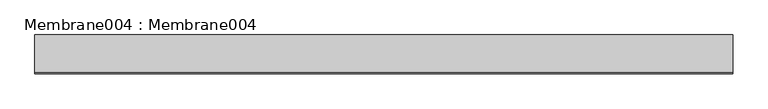
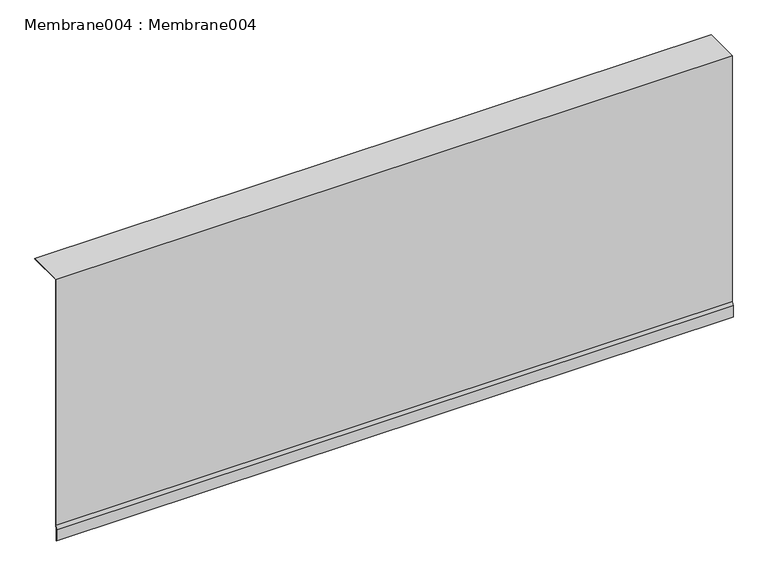
"""IFC4 building model written with IfcOpenShell, lengths in millimetres: proxy geometry, Membrane004 : Membrane004."""

from ifc_helpers import new_model, si_unit, frame, origin, place, context, project, spatial, polyline, outline, extrude, source, transform, mapped, element, save


def membrane004_membrane004_f78f7f05(model_context):
    return source(origin(), model_context, "Body", "SweptSolid", [
        extrude(outline(polyline([(-4304.4792138, 41057.992875), (-4304.4792138, 41056.992875), (-4410.2786824, 41056.992875), (-4410.2786824, 40289.0915624), (-4414.3643448, 40277.8662972), (-4414.3643448, 40242.9648437), (-4415.3643448, 40242.9648437), (-4415.3643448, 40278.0426242), (-4411.2786824, 40289.2678894), (-4411.2786824, 41057.992875), (-4304.4792138, 41057.992875)])), frame((12383.0178845, 0.0, 0.0), z_axis=(1.0, 0.0, 0.0), x_axis=(0.0, 1.0, 0.0)), (0.0, 0.0, 1.0), 2000.0),
    ])


if __name__ == "__main__":
    model = new_model("IFC4")
    model_context = context("Model", 3, world=origin())
    ifc_project = project(units=[si_unit("LENGTHUNIT", "METRE", prefix="MILLI")], contexts=[model_context])
    site = spatial("IfcSite", under=ifc_project)
    building = spatial("IfcBuilding", under=site)
    placement = place(None, origin())
    membrane004_membrane004_shape = membrane004_membrane004_f78f7f05(model_context)
    element("IfcBuildingElementProxy", 1, Name="Membrane004 : Membrane004", ObjectType="Membrane004 : Membrane004", at=placement, inside=building, context=model_context, shape_type="MappedRepresentation", body=[
        mapped(membrane004_membrane004_shape, transform((0.0, 0.0, 0.0), x_axis=(1.0, 0.0, 0.0), y_axis=(0.0, 1.0, 0.0), z_axis=(0.0, 0.0, 1.0))),
    ])
    save(model, "model.ifc")

# Revit data of these elements
# Type "Membrane004 : Membrane004"
#   NameOverride = "Membrane004"
# Element 1 (IfcBuildingElementProxy, "Membrane004 : Membrane004")
#   Materials on its faces: "2 LAYERS NO. 30 ASTM D226 ASPHALT SATURATED ORGANIC FELT"
# Materials
#   "2 LAYERS NO. 30 ASTM D226 ASPHALT SATURATED ORGANIC FELT": class "Unassigned", colour RGB 46 171 0, transparency 0
